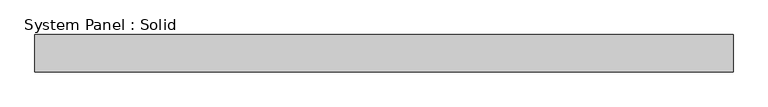
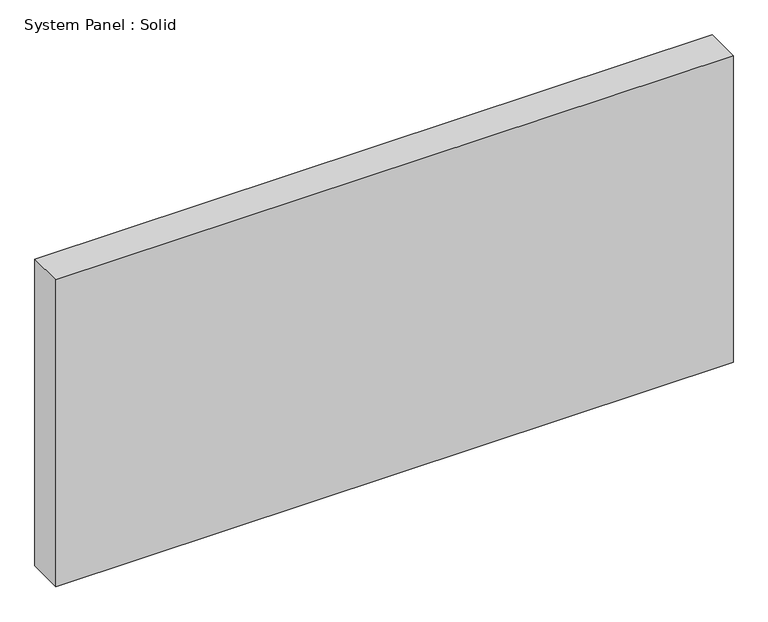
"""IFC4 building model written with IfcOpenShell, lengths in millimetres: plate geometry, System Panel : Solid."""

from ifc_helpers import new_model, si_unit, origin, origin_with_axes, place, context, project, spatial, polyline, outline, extrude, source, transform, mapped, element, save


def system_panel_solid_65092244(model_context):
    return source(origin(), model_context, "Body", "SweptSolid", [
        extrude(outline(polyline([(596.9, -19.05), (-596.9, -19.05), (-596.9, 44.45), (596.9, 44.45), (596.9, -19.05)])), origin_with_axes(), (0.0, 0.0, 1.0), 571.5),
    ])


if __name__ == "__main__":
    model = new_model("IFC4")
    model_context = context("Model", 3, world=origin())
    ifc_project = project(units=[si_unit("LENGTHUNIT", "METRE", prefix="MILLI")], contexts=[model_context])
    site = spatial("IfcSite", under=ifc_project)
    building = spatial("IfcBuilding", under=site)
    placement = place(None, origin())
    system_panel_solid_shape = system_panel_solid_65092244(model_context)
    element("IfcPlate", 1, ObjectType="System Panel : Solid", at=placement, inside=building, context=model_context, shape_type="MappedRepresentation", body=[
        mapped(system_panel_solid_shape, transform((0.0, 0.0, 0.0), x_axis=(1.0, 0.0, 0.0), y_axis=(0.0, 1.0, 0.0), z_axis=(0.0, 0.0, 1.0))),
    ])
    save(model, "model.ifc")

# Revit data of these elements
# Element 1 (IfcPlate, "System Panel : Solid")
#   Materials on its faces: "Default"
# Materials
#   "Default": class "Miscellaneous", colour RGB 127 127 127, transparency 0
